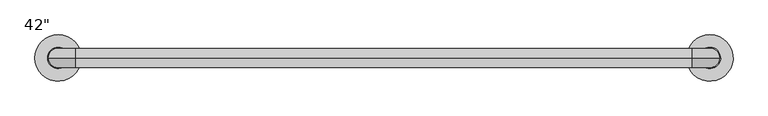
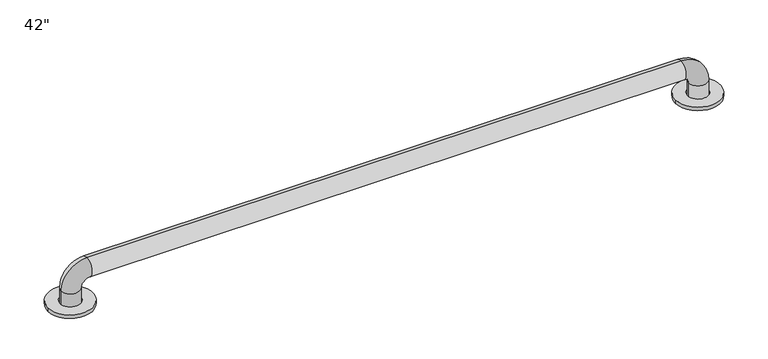
"""IFC4 building model written with IfcOpenShell, lengths in millimetres: proxy geometry."""

from ifc_helpers import new_model, si_unit, point, frame, frame_2d, origin, origin_with_axes, origin_2d, place, context, project, spatial, circle_curve, ellipse_curve, trimmed, segment, composite_curve, outline, extrude, source, transform, mapped, element, save
from ifc_brep_helpers import plane_surface, cylinder_surface, revolved_surface, advanced_brep


def proxy_594e2c3f(model_context):
    return source(origin(), model_context, "Body", "SolidModel", [
        extrude(outline(composite_curve([segment(trimmed(circle_curve(frame_2d((1066.8, 0.0)), 38.1), [point((1028.7, 0.0))], [point((1066.8, 38.1))], False, "CARTESIAN"), True, "CONTINUOUS"), segment(trimmed(circle_curve(frame_2d((1066.8, 0.0)), 38.1), [point((1066.8, 38.1))], [point((1028.7, 0.0))], False, "CARTESIAN"), True, "CONTINUOUS")], self_intersect=False), holes=[composite_curve([segment(trimmed(circle_curve(frame_2d((1066.8, 0.0)), 17.4625), [point((1049.3375, 0.0))], [point((1066.8, 17.4625))], True, "CARTESIAN"), True, "CONTINUOUS"), segment(trimmed(circle_curve(frame_2d((1066.8, 0.0)), 17.4625), [point((1066.8, 17.4625))], [point((1049.3375, 0.0))], True, "CARTESIAN"), True, "CONTINUOUS")], self_intersect=False)]), origin_with_axes(), (0.0, 0.0, 1.0), 6.35),
        extrude(outline(composite_curve([segment(trimmed(circle_curve(origin_2d(), 38.1), [point((-38.1, 0.0))], [point((0.0, 38.1))], False, "CARTESIAN"), True, "CONTINUOUS"), segment(trimmed(circle_curve(origin_2d(), 38.1), [point((0.0, 38.1))], [point((-38.1, 0.0))], False, "CARTESIAN"), True, "CONTINUOUS")], self_intersect=False), holes=[composite_curve([segment(trimmed(circle_curve(origin_2d(), 17.4625), [point((-17.4625, 0.0))], [point((0.0, 17.4625))], True, "CARTESIAN"), True, "CONTINUOUS"), segment(trimmed(circle_curve(origin_2d(), 17.4625), [point((0.0, 17.4625))], [point((-17.4625, 0.0))], True, "CARTESIAN"), True, "CONTINUOUS")], self_intersect=False)]), origin_with_axes(), (0.0, 0.0, 1.0), 6.35),
        advanced_brep(
        [(1082.675, 0.0, 0.0), (1050.925, 0.0, 0.0), (1050.925, 0.0, 28.575), (1082.675, 0.0, 28.575), (1038.225, 0.0, 41.275), (1038.225, 0.0, 73.025), (28.575, 0.0, 41.275), (28.575, 0.0, 73.025), (15.875, 0.0, 28.575), (-15.875, 0.0, 28.575), (-15.875, 0.0, 0.0), (15.875, 0.0, 0.0)],
        [
            (0, 1, circle_curve(frame((1066.8, 0.0, 0.0), z_axis=(0.0, 0.0, -1.0), x_axis=(-1.0, 0.0, 0.0)), 15.875)),
            (1, 0, circle_curve(frame((1066.8, 0.0, 0.0), z_axis=(0.0, 0.0, -1.0), x_axis=(-1.0, 0.0, 0.0)), 15.875)),
            (1, 2),
            (2, 3, circle_curve(frame((1066.8, 0.0, 28.575), z_axis=(0.0, 0.0, -1.0), x_axis=(-1.0, 0.0, 0.0)), 15.875)),
            (3, 0),
            (3, 2, circle_curve(frame((1066.8, 0.0, 28.575), z_axis=(0.0, 0.0, -1.0), x_axis=(-1.0, 0.0, 0.0)), 15.875)),
            (4, 5, circle_curve(frame((1038.225, 0.0, 57.15), z_axis=(1.0, 0.0, 0.0), x_axis=(0.0, 0.0, -1.0)), 15.875)),
            (5, 3, circle_curve(frame((1038.225, 0.0, 28.575), z_axis=(0.0, 1.0, 0.0), x_axis=(1.0, 0.0, 0.0)), 44.45)),
            (2, 4, circle_curve(frame((1038.225, 0.0, 28.575), z_axis=(0.0, -1.0, 0.0), x_axis=(1.0, 0.0, 0.0)), 12.7)),
            (5, 4, circle_curve(frame((1038.225, 0.0, 57.15), z_axis=(1.0, 0.0, 0.0), x_axis=(0.0, 0.0, -1.0)), 15.875)),
            (4, 6),
            (6, 7, circle_curve(frame((28.575, 0.0, 57.15), z_axis=(1.0, 0.0, 0.0), x_axis=(0.0, 0.0, -1.0)), 15.875)),
            (7, 5),
            (7, 6, circle_curve(frame((28.575, 0.0, 57.15), z_axis=(1.0, 0.0, 0.0), x_axis=(0.0, 0.0, -1.0)), 15.875)),
            (8, 9, circle_curve(frame((0.0, 0.0, 28.575), z_axis=(0.0, 0.0, 1.0), x_axis=(1.0, 0.0, 0.0)), 15.875)),
            (9, 7, circle_curve(frame((28.575, 0.0, 28.575), z_axis=(0.0, 1.0, 0.0), x_axis=(0.0, 0.0, 1.0)), 44.45)),
            (6, 8, circle_curve(frame((28.575, 0.0, 28.575), z_axis=(0.0, -1.0, 0.0), x_axis=(0.0, 0.0, 1.0)), 12.7)),
            (9, 8, circle_curve(frame((0.0, 0.0, 28.575), z_axis=(0.0, 0.0, 1.0), x_axis=(1.0, 0.0, 0.0)), 15.875)),
            (10, 11, circle_curve(frame((0.0, 0.0, 0.0), z_axis=(0.0, 0.0, -1.0), x_axis=(1.0, 0.0, 0.0)), 15.875)),
            (11, 10, circle_curve(frame((0.0, 0.0, 0.0), z_axis=(0.0, 0.0, -1.0), x_axis=(1.0, 0.0, 0.0)), 15.875)),
            (8, 11),
            (10, 9),
        ],
        [
            plane_surface(frame((1066.8, 0.0, 0.0), z_axis=(0.0, 0.0, -1.0), x_axis=(0.0, 1.0, 0.0))),
            cylinder_surface(frame((1066.8, 0.0, 0.0), z_axis=(0.0, 0.0, -1.0), x_axis=(-1.0, 0.0, 0.0)), 15.875),
            revolved_surface(trimmed(ellipse_curve(frame((1066.8, 0.0, 28.575), z_axis=(0.0, 0.0, 1.0), x_axis=(-1.0, 0.0, 0.0)), 15.875, 15.875), [point((1082.675, 0.0, 28.575))], [point((1050.925, 0.0, 28.575))], True, "CARTESIAN"), (1038.225, 0.0, 28.575), (0.0, 1.0, 0.0)),
            revolved_surface(trimmed(ellipse_curve(frame((1066.8, 0.0, 28.575), z_axis=(0.0, 0.0, 1.0), x_axis=(-1.0, 0.0, 0.0)), 15.875, 15.875), [point((1050.925, 0.0, 28.575))], [point((1082.675, 0.0, 28.575))], True, "CARTESIAN"), (1038.225, 0.0, 28.575), (0.0, 1.0, 0.0)),
            cylinder_surface(frame((1038.225, 0.0, 57.15), z_axis=(1.0, 0.0, 0.0), x_axis=(0.0, 0.0, -1.0)), 15.875),
            revolved_surface(trimmed(ellipse_curve(frame((28.575, 0.0, 57.15), z_axis=(-1.0, 0.0, 0.0), x_axis=(0.0, 0.0, -1.0)), 15.875, 15.875), [point((28.575, 0.0, 73.025))], [point((28.575, 0.0, 41.275))], True, "CARTESIAN"), (28.575, 0.0, 28.575), (0.0, 1.0, 0.0)),
            revolved_surface(trimmed(ellipse_curve(frame((28.575, 0.0, 57.15), z_axis=(-1.0, 0.0, 0.0), x_axis=(0.0, 0.0, -1.0)), 15.875, 15.875), [point((28.575, 0.0, 41.275))], [point((28.575, 0.0, 73.025))], True, "CARTESIAN"), (28.575, 0.0, 28.575), (0.0, 1.0, 0.0)),
            plane_surface(frame((0.0, 0.0, 0.0), z_axis=(0.0, 0.0, -1.0), x_axis=(0.0, 1.0, 0.0))),
            cylinder_surface(frame((0.0, 0.0, 28.575), z_axis=(0.0, 0.0, 1.0), x_axis=(1.0, 0.0, 0.0)), 15.875),
        ],
        [
            (0, [[1, 2]]),
            (1, [[3, 4, 5, -2]]),
            (1, [[-5, 6, -3, -1]]),
            (2, [[7, 8, -4, 9]]),
            (3, [[10, -9, -6, -8]]),
            (4, [[11, 12, 13, -7]]),
            (4, [[-13, 14, -11, -10]]),
            (5, [[15, 16, -12, 17]]),
            (6, [[18, -17, -14, -16]]),
            (7, [[19, 20]]),
            (8, [[21, -19, 22, -15]]),
            (8, [[-22, -20, -21, -18]]),
        ],
    ),
    ])


if __name__ == "__main__":
    model = new_model("IFC4")
    model_context = context("Model", 3, world=origin())
    ifc_project = project(units=[si_unit("LENGTHUNIT", "METRE", prefix="MILLI")], contexts=[model_context])
    site = spatial("IfcSite", under=ifc_project)
    building = spatial("IfcBuilding", under=site)
    placement = place(None, origin())
    proxy_shape = proxy_594e2c3f(model_context)
    element("IfcBuildingElementProxy", 1, Name="Seqm-Grab Bar : 42\"", ObjectType="Seqm-Grab Bar : 42\"", at=placement, inside=building, context=model_context, shape_type="MappedRepresentation", body=[
        mapped(proxy_shape, transform((0.0, 0.0, 0.0), x_axis=(1.0, 0.0, 0.0), y_axis=(0.0, 1.0, 0.0), z_axis=(0.0, 0.0, 1.0))),
    ])
    save(model, "model.ifc")

# Revit data of these elements
# Type "Seqm-Grab Bar : 42\""
#   Spec Number = "10 28 00"
#   Spec Description = "42\" GRAB BAR"
#   Length = 3' - 6"
#   Default Elevation = 4' - 0"
#   Grab Bar Material = GRAB BARS - AT ADA RESTROOMS ONLY
# Element 1 (IfcBuildingElementProxy, "Seqm-Grab Bar : 42\"")
#   Materials on its faces: "GRAB BARS - AT ADA RESTROOMS ONLY"
# Materials
#   "GRAB BARS - AT ADA RESTROOMS ONLY": class "Generic", colour RGB 120 120 120, transparency 0, Cost = 0
